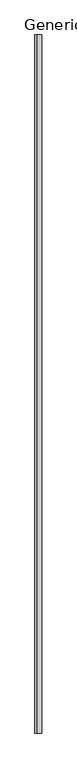
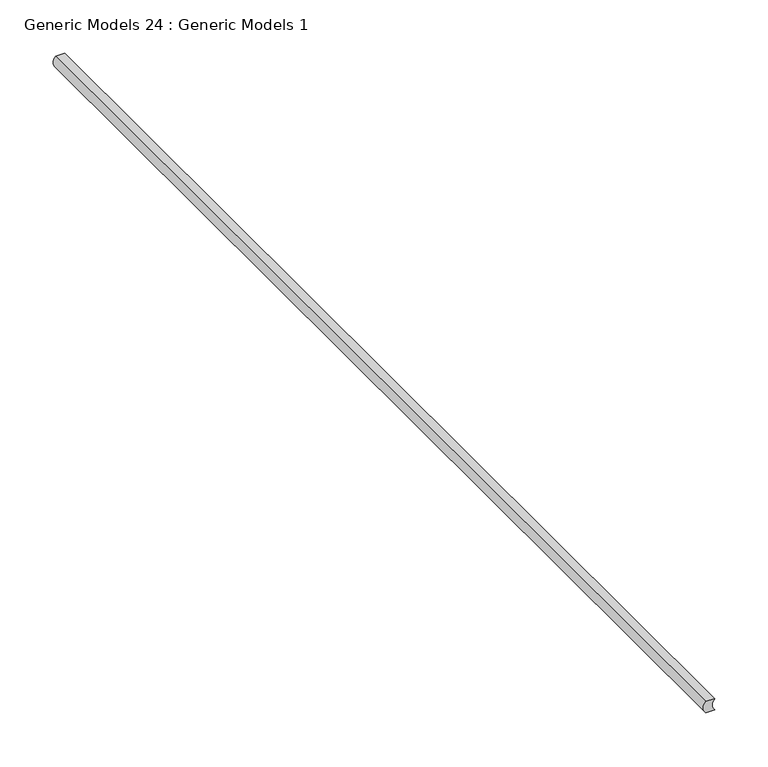
"""IFC4 building model written with IfcOpenShell, lengths in millimetres: proxy geometry, Generic Models 24 : Generic Models 1."""

import ifcopenshell
import ifcopenshell.guid

model = None  # the IFC model being written
_history = None  # IfcOwnerHistory: only IFC2X3 demands one
_inside = {}  # id of a spatial element -> (the spatial element, [elements in it])
_under = {}  # id of a project, library or spatial element -> (it, [spatial elements below it])
_declared = {}  # id of a project -> (the project, [libraries it declares])
_typed = {}  # id of a type object -> (the type object, [elements of that type])
_made_of = {}  # id of a material, layer set ... -> (it, [elements and type objects made of it])


def new_model(schema):
    """Start an empty IFC model of exactly this schema.

    Asked for "IFC4X3", IfcOpenShell would pick the latest addendum, in which some entities
    have other attributes; the version numbers below select the first issue.
    IFC2X3 requires an IfcOwnerHistory on every rooted entity: one is made here for all.
    """
    global model, _history
    if schema == "IFC4X3":
        model = ifcopenshell.file(schema_version=(4, 3, 0, 0))
    else:
        model = ifcopenshell.file(schema=schema)
    _inside.clear()
    _under.clear()
    _declared.clear()
    _typed.clear()
    _made_of.clear()
    _history = None
    if model.schema == "IFC2X3":
        org = make("IfcOrganization", Name="unknown")
        user = make(
            "IfcPersonAndOrganization",
            ThePerson=make("IfcPerson", FamilyName="unknown"),
            TheOrganization=org,
        )
        app = make(
            "IfcApplication",
            ApplicationDeveloper=org,
            Version="unknown",
            ApplicationFullName="unknown",
            ApplicationIdentifier="unknown",
        )
        _history = make(
            "IfcOwnerHistory",
            OwningUser=user,
            OwningApplication=app,
            ChangeAction="ADDED",
            CreationDate=0,
        )
    return model


def make(cls, **values):
    """One entity of the class cls with the attributes given. An attribute that is None is left unset."""
    return model.create_entity(
        cls, **{name: value for name, value in values.items() if value is not None}
    )


def rooted(cls, **values):
    """An entity with a GlobalId (a new one), such as an element, a storey or a relation."""
    return make(cls, GlobalId=ifcopenshell.guid.new(), OwnerHistory=_history, **values)


def si_unit(unit_type, name, prefix=None):
    """IfcSIUnit, for example si_unit("LENGTHUNIT", "METRE", prefix="MILLI")."""
    return make("IfcSIUnit", UnitType=unit_type, Prefix=prefix, Name=name)


def assignment(units):
    """IfcUnitAssignment: the units of a project."""
    return None if units is None else make("IfcUnitAssignment", Units=units)


def point(xyz):
    """IfcCartesianPoint."""
    return None if xyz is None else make("IfcCartesianPoint", Coordinates=xyz)


def direction(xyz):
    """IfcDirection."""
    return None if xyz is None else make("IfcDirection", DirectionRatios=xyz)


def frame(location, z_axis=None, x_axis=None):
    """IfcAxis2Placement3D, a coordinate frame: its origin and axes. An axis left out is left unset."""
    return make(
        "IfcAxis2Placement3D",
        Location=point(location),
        Axis=direction(z_axis),
        RefDirection=direction(x_axis),
    )


def frame_2d(location, x_axis=None):
    """IfcAxis2Placement2D, a coordinate frame in the plane: its origin and x axis."""
    return make(
        "IfcAxis2Placement2D", Location=point(location), RefDirection=direction(x_axis)
    )


def origin():
    """The frame at (0, 0, 0) with its axes left unset."""
    return frame((0.0, 0.0, 0.0))


def place(relative_to, where):
    """IfcLocalPlacement: puts the frame where relative to a parent placement (None: the world)."""
    return make(
        "IfcLocalPlacement", PlacementRelTo=relative_to, RelativePlacement=where
    )


def context(
    kind, dimensions, precision=None, world=None, true_north=None, identifier=None
):
    """IfcGeometricRepresentationContext, for example the 3D "Model" context."""
    return make(
        "IfcGeometricRepresentationContext",
        ContextIdentifier=identifier,
        ContextType=kind,
        CoordinateSpaceDimension=dimensions,
        Precision=precision,
        WorldCoordinateSystem=world,
        TrueNorth=true_north,
    )


def project(units=None, contexts=None):
    """IfcProject with its units and contexts."""
    return rooted(
        "IfcProject",
        Name="project",
        RepresentationContexts=contexts,
        UnitsInContext=assignment(units),
    )


def spatial(cls, under=None, at=None, **own):
    """A site, building, storey or space (cls), placed at a placement, below another one or the project."""
    s = rooted(cls, ObjectPlacement=at, **own)
    if under is not None:
        _under.setdefault(under.id(), (under, []))[1].append(s)
    return s


def polyline(points):
    """IfcPolyline through the points."""
    return make("IfcPolyline", Points=[point(p) for p in points])


def circle_curve(where, radius):
    """IfcCircle in the frame where."""
    return make("IfcCircle", Position=where, Radius=radius)


def trimmed(basis, trim1, trim2, sense, master):
    """IfcTrimmedCurve: the piece of a basis curve between two trims."""
    return make(
        "IfcTrimmedCurve",
        BasisCurve=basis,
        Trim1=trim1,
        Trim2=trim2,
        SenseAgreement=sense,
        MasterRepresentation=master,
    )


def segment(curve, same_sense, transition):
    """IfcCompositeCurveSegment."""
    return make(
        "IfcCompositeCurveSegment",
        Transition=transition,
        SameSense=same_sense,
        ParentCurve=curve,
    )


def composite_curve(segments, self_intersect=None):
    """IfcCompositeCurve: segments joined end to end."""
    return make("IfcCompositeCurve", Segments=segments, SelfIntersect=self_intersect)


def outline(outer, holes=None, kind="AREA"):
    """IfcArbitraryClosedProfileDef: a profile drawn as a closed curve; with holes, ...WithVoids."""
    if holes is None:
        return make("IfcArbitraryClosedProfileDef", ProfileType=kind, OuterCurve=outer)
    return make(
        "IfcArbitraryProfileDefWithVoids",
        ProfileType=kind,
        OuterCurve=outer,
        InnerCurves=holes,
    )


def extrude(swept, where, along, depth):
    """IfcExtrudedAreaSolid: the profile swept, set in the frame where, extruded along a direction by depth."""
    return make(
        "IfcExtrudedAreaSolid",
        SweptArea=swept,
        Position=where,
        ExtrudedDirection=direction(along),
        Depth=depth,
    )


def shape(context_of_items, identifier, shape_type, items):
    """IfcShapeRepresentation: the items that make up one representation, for example the "Body"."""
    return make(
        "IfcShapeRepresentation",
        ContextOfItems=context_of_items,
        RepresentationIdentifier=identifier,
        RepresentationType=shape_type,
        Items=items,
    )


def source(mapping_origin, context_of_items, identifier, shape_type, items):
    """IfcRepresentationMap: a shape defined once, which mapped items show again and again."""
    return make(
        "IfcRepresentationMap",
        MappingOrigin=mapping_origin,
        MappedRepresentation=shape(context_of_items, identifier, shape_type, items),
    )


def transform(
    local_origin,
    x_axis=None,
    y_axis=None,
    z_axis=None,
    scale=None,
    scale2=None,
    scale3=None,
    uniform=True,
):
    """IfcCartesianTransformationOperator3D, or its non-uniform kind. x_axis, y_axis, z_axis: its Axis1, 2, 3."""
    if uniform:
        return make(
            "IfcCartesianTransformationOperator3D",
            Axis1=direction(x_axis),
            Axis2=direction(y_axis),
            LocalOrigin=point(local_origin),
            Scale=scale,
            Axis3=direction(z_axis),
        )
    return make(
        "IfcCartesianTransformationOperator3DnonUniform",
        Axis1=direction(x_axis),
        Axis2=direction(y_axis),
        LocalOrigin=point(local_origin),
        Scale=scale,
        Axis3=direction(z_axis),
        Scale2=scale2,
        Scale3=scale3,
    )


def mapped(mapping_source, mapping_target):
    """IfcMappedItem: shows the shape of a source again, moved by a transform."""
    return make(
        "IfcMappedItem", MappingSource=mapping_source, MappingTarget=mapping_target
    )


def made_of(thing, what):
    """Note that an element or type object is made of a material, layer set ...; save() writes the relation."""
    if what is not None:
        _made_of.setdefault(what.id(), (what, []))[1].append(thing)
    return thing


def element(
    cls,
    number,
    at=None,
    inside=None,
    cuts=None,
    type_object=None,
    material=None,
    context=None,
    identifier="Body",
    shape_type=None,
    held_by="IfcProductDefinitionShape",
    body=None,
    shapes=None,
    **own,
):
    """One element of the class cls, such as IfcWall. Its Tag is "e" and its number.

    at: its placement. inside: the storey or other place that contains it. cuts: it is an
    opening in that element (IfcRelVoidsElement). A single representation is given by context,
    identifier, shape_type and body (its items); several are given by shapes. held_by: the class
    of the entity that holds the representations. save() writes the other relations.
    """
    e = rooted(cls, Tag="e%d" % number, ObjectPlacement=at, **own)
    if body is not None:
        shapes = [shape(context, identifier, shape_type, body)]
    if shapes is not None:
        e.Representation = make(held_by, Representations=shapes)
    if inside is not None:
        _inside.setdefault(inside.id(), (inside, []))[1].append(e)
    if cuts is not None:
        rooted(
            "IfcRelVoidsElement", RelatingBuildingElement=cuts, RelatedOpeningElement=e
        )
    if type_object is not None:
        _typed.setdefault(type_object.id(), (type_object, []))[1].append(e)
    return made_of(e, material)


def aggregate(whole, parts):
    """IfcRelAggregates: a whole, such as a stair, and the parts it consists of."""
    return rooted("IfcRelAggregates", RelatingObject=whole, RelatedObjects=parts)


def save(model, path):
    """Write the relations noted so far, then the file.

    IfcRelAggregates (storeys below a building ...), IfcRelContainedInSpatialStructure (elements
    in a storey), IfcRelDefinesByType, IfcRelAssociatesMaterial and IfcRelDeclares: one each for
    every whole, place, type object, material and project.
    """
    for whole, parts in _under.values():
        aggregate(whole, parts)
    for where, things in _inside.values():
        rooted(
            "IfcRelContainedInSpatialStructure",
            RelatedElements=things,
            RelatingStructure=where,
        )
    for kind, things in _typed.values():
        rooted("IfcRelDefinesByType", RelatedObjects=things, RelatingType=kind)
    for what, things in _made_of.values():
        rooted("IfcRelAssociatesMaterial", RelatedObjects=things, RelatingMaterial=what)
    for by, libraries in _declared.values():
        rooted("IfcRelDeclares", RelatingContext=by, RelatedDefinitions=libraries)
    model.write(path)


def generic_models_24_generic_models_1_a9595ea3(model_context):
    return source(origin(), model_context, "Body", "SweptSolid", [
        extrude(outline(composite_curve([segment(trimmed(circle_curve(frame_2d((2451.1, 49805.704481)), 8.620055), [point((2444.75, 49799.875))], [point((2457.45, 49799.875))], True, "CARTESIAN"), True, "CONTINUOUS"), segment(polyline([(2457.45, 49799.875), (2457.45, 49790.35)]), True, "CONTINUOUS"), segment(trimmed(circle_curve(frame_2d((2451.1, 49796.179481)), 8.620055), [point((2457.45, 49790.35))], [point((2444.75, 49790.35))], False, "CARTESIAN"), True, "CONTINUOUS"), segment(polyline([(2444.75, 49790.35), (2444.75, 49799.875)]), True, "CONTINUOUS")], self_intersect=False)), frame((0.0, 0.0, 0.0), z_axis=(0.0, 1.0, 0.0), x_axis=(0.0, 0.0, 1.0)), (0.0, 0.0, 1.0), 1219.2),
    ])


if __name__ == "__main__":
    model = new_model("IFC4")
    model_context = context("Model", 3, world=origin())
    ifc_project = project(units=[si_unit("LENGTHUNIT", "METRE", prefix="MILLI")], contexts=[model_context])
    site = spatial("IfcSite", under=ifc_project)
    building = spatial("IfcBuilding", under=site)
    placement = place(None, origin())
    generic_models_24_generic_models_1_shape = generic_models_24_generic_models_1_a9595ea3(model_context)
    element("IfcBuildingElementProxy", 1, Name="Generic Models 24 : Generic Models 1", ObjectType="Generic Models 24 : Generic Models 1", at=placement, inside=building, context=model_context, shape_type="MappedRepresentation", body=[
        mapped(generic_models_24_generic_models_1_shape, transform((0.0, 0.0, 0.0), x_axis=(1.0, 0.0, 0.0), y_axis=(0.0, 1.0, 0.0), z_axis=(0.0, 0.0, 1.0))),
    ])
    save(model, "model.ifc")

# Revit data of these elements
# Element 1 (IfcBuildingElementProxy, "Generic Models 24 : Generic Models 1")
#   Materials on its faces: "ACOUSTICAL SEALANT"
# Materials
#   "ACOUSTICAL SEALANT": class "Unassigned", colour RGB 120 120 120, transparency 0, Cost = 0
